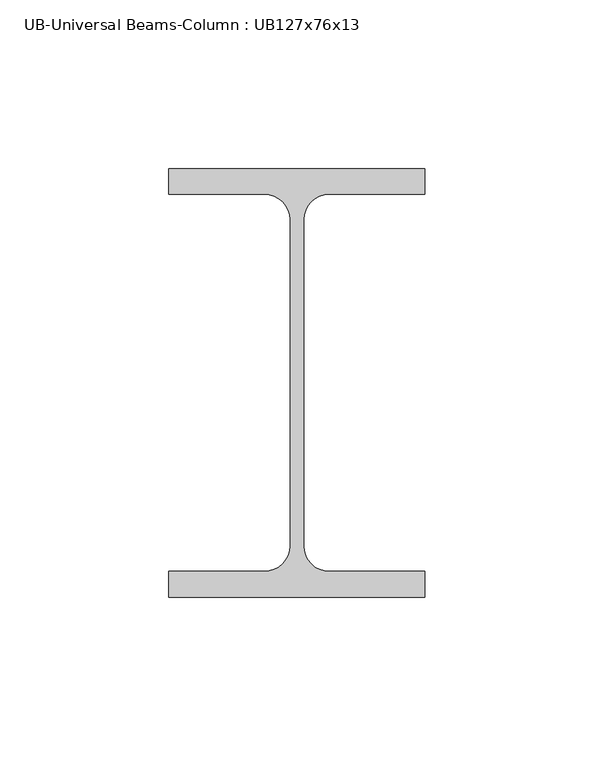
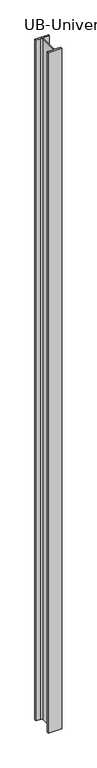
"""IFC4 building model written with IfcOpenShell, lengths in millimetres: column geometry, UB-Universal Beams-Column : UB127x76x13."""

from ifc_helpers import new_model, si_unit, point, frame_2d, origin, origin_with_axes, place, context, project, spatial, polyline, circle_curve, trimmed, segment, composite_curve, outline, extrude, source, transform, mapped, element, save


def ub_universal_beams_column_ub127x76x13_3e05bf5d(model_context):
    return source(origin(), model_context, "Body", "SweptSolid", [
        extrude(outline(composite_curve([segment(polyline([(38.0, 63.5), (38.0, 55.9), (9.6, 55.9)]), True, "CONTINUOUS"), segment(trimmed(circle_curve(frame_2d((9.6, 48.3)), 7.6), [point((9.6, 55.9))], [point((2.0, 48.3))], True, "CARTESIAN"), True, "CONTINUOUS"), segment(polyline([(2.0, 48.3), (2.0, -48.3)]), True, "CONTINUOUS"), segment(trimmed(circle_curve(frame_2d((9.6, -48.3)), 7.6), [point((2.0, -48.3))], [point((9.6, -55.9))], True, "CARTESIAN"), True, "CONTINUOUS"), segment(polyline([(9.6, -55.9), (38.0, -55.9), (38.0, -63.5), (-38.0, -63.5), (-38.0, -55.9), (-9.6, -55.9)]), True, "CONTINUOUS"), segment(trimmed(circle_curve(frame_2d((-9.6, -48.3)), 7.6), [point((-9.6, -55.9))], [point((-2.0, -48.3))], True, "CARTESIAN"), True, "CONTINUOUS"), segment(polyline([(-2.0, -48.3), (-2.0, 48.3)]), True, "CONTINUOUS"), segment(trimmed(circle_curve(frame_2d((-9.6, 48.3)), 7.6), [point((-2.0, 48.3))], [point((-9.6, 55.9))], True, "CARTESIAN"), True, "CONTINUOUS"), segment(polyline([(-9.6, 55.9), (-38.0, 55.9), (-38.0, 63.5), (38.0, 63.5)]), True, "CONTINUOUS")], self_intersect=False)), origin_with_axes(), (0.0, 0.0, 1.0), 4000.0),
    ])


if __name__ == "__main__":
    model = new_model("IFC4")
    model_context = context("Model", 3, world=origin())
    ifc_project = project(units=[si_unit("LENGTHUNIT", "METRE", prefix="MILLI")], contexts=[model_context])
    site = spatial("IfcSite", under=ifc_project)
    building = spatial("IfcBuilding", under=site)
    placement = place(None, origin())
    ub_universal_beams_column_ub127x76x13_shape = ub_universal_beams_column_ub127x76x13_3e05bf5d(model_context)
    element("IfcColumn", 1, ObjectType="UB-Universal Beams-Column : UB127x76x13", at=placement, inside=building, context=model_context, shape_type="MappedRepresentation", body=[
        mapped(ub_universal_beams_column_ub127x76x13_shape, transform((0.0, 0.0, 0.0), x_axis=(1.0, 0.0, 0.0), y_axis=(0.0, 1.0, 0.0), z_axis=(0.0, 0.0, 1.0))),
    ])
    save(model, "model.ifc")

# Revit data of these elements
# Type "UB-Universal Beams-Column : UB127x76x13"
#   Section Name Key = "UB127X76X13"
#   Width = 7.6 cm
#   Web Thickness = 0.4 cm
#   Web Fillet = 0.76 cm
#   Warping Constant = 2000.0 cm⁶
#   Torsional Moment of Inertia = 2.85 cm⁴
#   Section Area = 16.5 cm²
#   Plastic Modulus weak axis = 22.6 cm³
#   Plastic Modulus strong axis = 84.2 cm³
#   Nominal Weight = 13.00 kgf/m
#   Moment of Inertia weak axis = 55.70 cm⁴
#   Moment of Inertia strong axis = 473.00 cm⁴
#   Height = 12.7 cm
#   Flange Thickness = 0.76 cm
#   Elastic Modulus weak axis = 14.7 cm³
#   Elastic Modulus strong axis = 74.6 cm³
#   Centroid Vertical = 6.35 cm
#   Centroid Horizontal = 3.8 cm
#   Bolt Spacing = 4.0 cm
#   Structural Material [instance default] = Metal - Steel 43-275
#   Type Comments = ""
#   Assembly Code = ""
# Element 1 (IfcColumn, "UB-Universal Beams-Column : UB127x76x13")
#   Materials on its faces: "Metal - Steel 43-275"
# Materials
#   "Metal - Steel 43-275": class "Metal", colour RGB 247 247 247, transparency 0, Cost = 0
